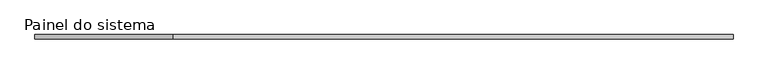
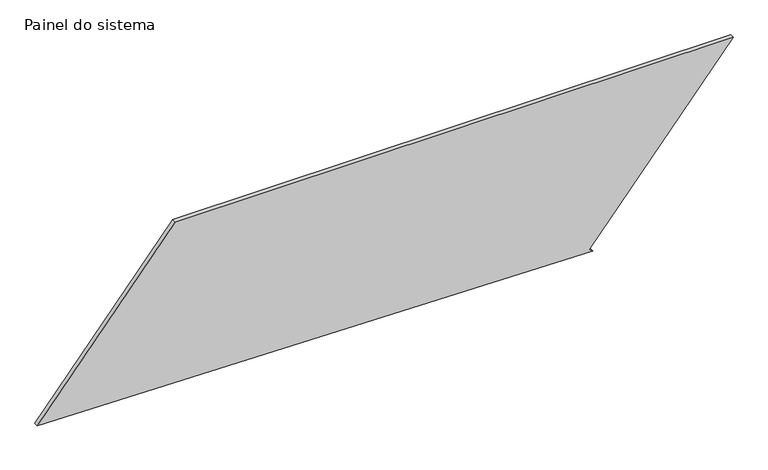
"""IFC4 building model written with IfcOpenShell, lengths in millimetres: plate geometry, Painel do sistema : Envidraçado."""

from ifc_helpers import new_model, si_unit, frame, origin, place, context, project, spatial, polyline, outline, extrude, source, transform, mapped, element, save


def painel_do_sistema_4524a12a(model_context):
    return source(origin(), model_context, "Body", "SweptSolid", [
        extrude(outline(polyline([(0.0, 1227.6841864), (15.8992441, 1208.391337), (1047.6971112, 2058.6963299), (1047.6971112, -1242.5642867), (57.36622, -2058.6963299), (0.0, 1227.6841864)])), frame((0.0, 24.5, 0.0), z_axis=(0.0, 1.0, 0.0), x_axis=(0.0, 0.0, 1.0)), (0.0, 0.0, 1.0), 25.0),
    ])


if __name__ == "__main__":
    model = new_model("IFC4")
    model_context = context("Model", 3, world=origin())
    ifc_project = project(units=[si_unit("LENGTHUNIT", "METRE", prefix="MILLI")], contexts=[model_context])
    site = spatial("IfcSite", under=ifc_project)
    building = spatial("IfcBuilding", under=site)
    placement = place(None, origin())
    painel_do_sistema_shape = painel_do_sistema_4524a12a(model_context)
    element("IfcPlate", 1, ObjectType="Painel do sistema : Envidraçado", at=placement, inside=building, context=model_context, shape_type="MappedRepresentation", body=[
        mapped(painel_do_sistema_shape, transform((0.0, 0.0, 0.0), x_axis=(1.0, 0.0, 0.0), y_axis=(0.0, 1.0, 0.0), z_axis=(0.0, 0.0, 1.0))),
    ])
    save(model, "model.ifc")

# Revit data of these elements
# Type "Painel do sistema : Envidraçado"
#   Construction Type Id = "GSP4R"
#   Analytic Construction = "Vidraça única Pilkington 1/8 pol"
#   Visual Light Transmittance = 0.9
#   Solar Heat Gain Coefficient = 0.86
#   Heat Transfer Coefficient (U) = 6.7069 W/(m²·K)
# Element 1 (IfcPlate, "Painel do sistema : Envidraçado")
#   Materials on its faces: "Vidro"
# Materials
#   "Vidro": class "Vidro", colour RGB 0 128 192, transparency 0.9, Description = "Vidro de sílica", Cost = 0
